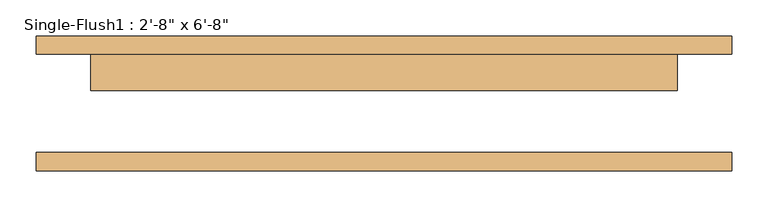
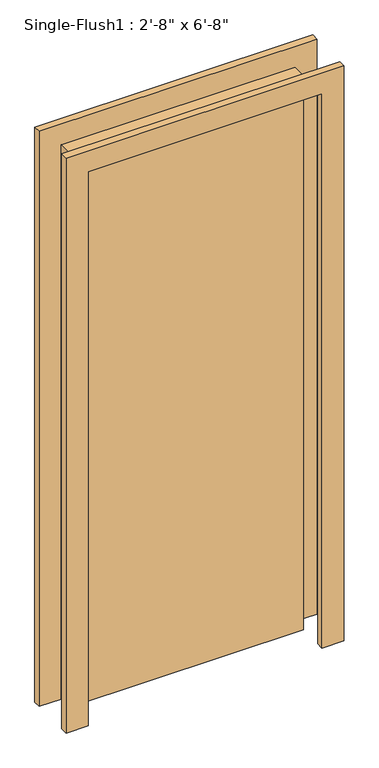
"""IFC4 building model written with IfcOpenShell, lengths in millimetres: door geometry."""

from ifc_helpers import new_model, si_unit, frame, origin, origin_with_axes, place, context, project, spatial, polyline, outline, extrude, source, transform, mapped, element, save


def door_2fa8c1c4(model_context):
    return source(origin(), model_context, "Body", "SweptSolid", [
        extrude(outline(polyline([(2108.2, -482.6), (0.0, -482.6), (0.0, -406.4), (2032.0, -406.4), (2032.0, 406.4), (0.0, 406.4), (0.0, 482.6), (2108.2, 482.6), (2108.2, -482.6)])), frame((0.0, 68.2625, 0.0), z_axis=(0.0, 1.0, 0.0), x_axis=(0.0, 0.0, 1.0)), (0.0, 0.0, 1.0), 25.4),
        extrude(outline(polyline([(2108.2, 482.6), (2108.2, -482.6), (0.0, -482.6), (0.0, -406.4), (2032.0, -406.4), (2032.0, 406.4), (0.0, 406.4), (0.0, 482.6), (2108.2, 482.6)])), frame((0.0, -93.6625, 0.0), z_axis=(0.0, 1.0, 0.0), x_axis=(0.0, 0.0, 1.0)), (0.0, 0.0, 1.0), 25.4),
        extrude(outline(polyline([(406.4, 17.4625), (-406.4, 17.4625), (-406.4, 68.2625), (406.4, 68.2625), (406.4, 17.4625)])), origin_with_axes(), (0.0, 0.0, 1.0), 2032.0),
    ])


if __name__ == "__main__":
    model = new_model("IFC4")
    model_context = context("Model", 3, world=origin())
    ifc_project = project(units=[si_unit("LENGTHUNIT", "METRE", prefix="MILLI")], contexts=[model_context])
    site = spatial("IfcSite", under=ifc_project)
    building = spatial("IfcBuilding", under=site)
    placement = place(None, origin())
    door_shape = door_2fa8c1c4(model_context)
    element("IfcDoor", 1, ObjectType="Single-Flush1 : 2'-8\" x 6'-8\"", at=placement, inside=building, context=model_context, shape_type="MappedRepresentation", body=[
        mapped(door_shape, transform((0.0, 0.0, 0.0), x_axis=(1.0, 0.0, 0.0), y_axis=(0.0, 1.0, 0.0), z_axis=(0.0, 0.0, 1.0))),
    ])
    save(model, "model.ifc")

# Revit data of these elements
# Type "Single-Flush1 : 2'-8\" x 6'-8\""
#   Type Mark = "D4"
#   Construction Type Id = "MDOOR"
#   Assembly Code = "C1020"
#   Analytic Construction = "Metal"
#   Thickness = 0' - 2"
#   Heat Transfer Coefficient (U) = 3.7021 W/(m²·K)
#   Height = 6' - 8"
#   Trim Projection Ext = 0' - 1"
#   Trim Projection Int = 0' - 1"
#   Trim Width = 0' - 3"
#   Width = 2' - 8"
#   Door Material = Door - Panel
#   Frame Material = Door - Frame
#   Visual Light Transmittance = 0
#   Solar Heat Gain Coefficient = 0
#   Function = (empty or 0)
#   Wall Closure = (empty or 0)
# Element 1 (IfcDoor, "Single-Flush1 : 2'-8\" x 6'-8\"")
#   Materials on its faces: "Door - Frame", "Door - Panel"
# Materials
#   "Door - Panel": class "Wood", colour RGB 210 159 95, transparency 0, Cost = 0
#   "Door - Frame": class "Miscellaneous", colour RGB 118 70 51, transparency 0, Cost = 0
